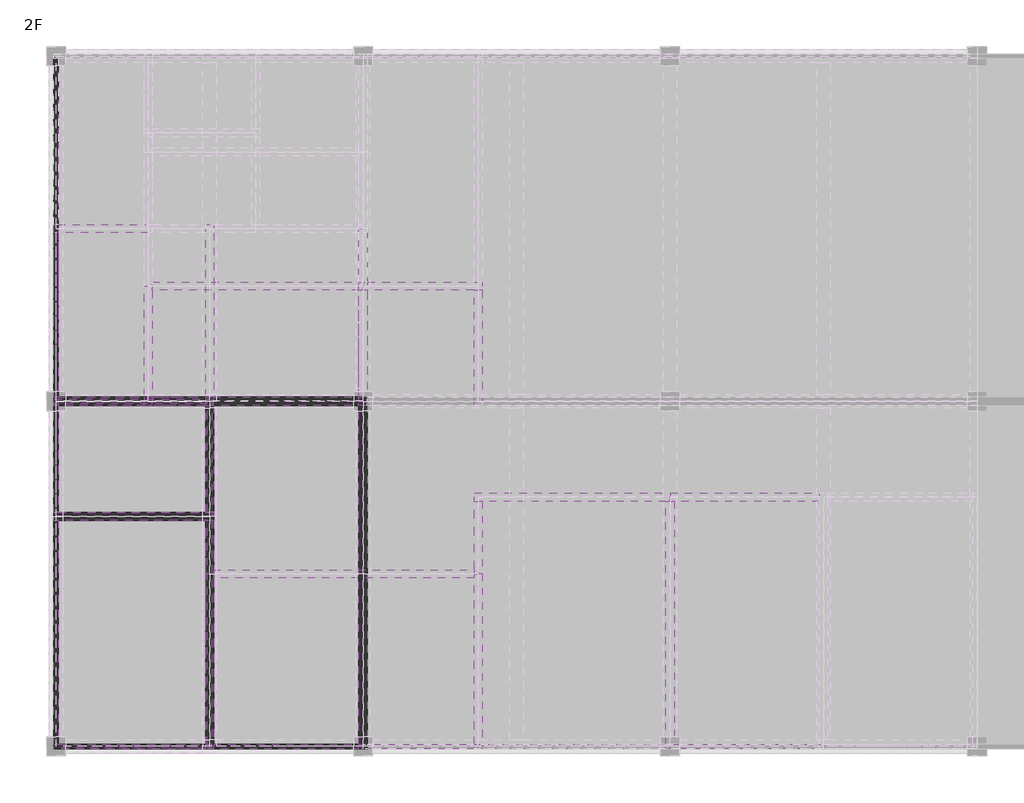
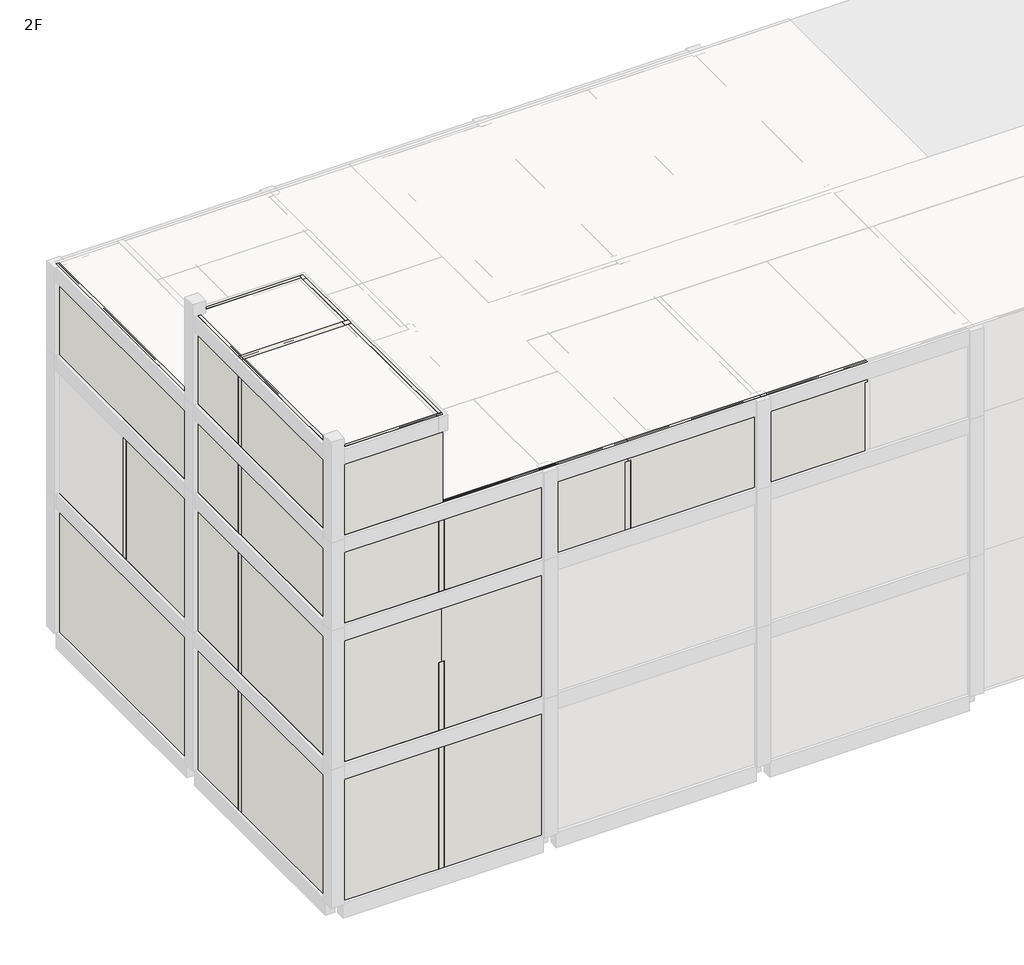
# One storey, part 1 of 7: 56 walls.
"""IFC4 building model written with IfcOpenShell, lengths in millimetres."""

from ifc_helpers import new_model, si_unit, frame, origin, place, context, project, spatial, polyline, outline, extrude, faceted_brep, element, save

model = new_model("IFC4")

# Units and contexts
model_context = context("Model", 3, world=origin())
ifc_project = project(units=[si_unit("LENGTHUNIT", "METRE", prefix="MILLI")], contexts=[model_context])

# Site, building, storey
site = spatial("IfcSite", under=ifc_project)
building = spatial("IfcBuilding", under=site)
storey = spatial("IfcBuildingStorey", under=building, Name="2F", Elevation=3500.0)

# Walls
placement = place(None, origin())
element("IfcWall", 1, ObjectType="WA211_Exterior-Cement Brick-90mm", at=placement, inside=storey, context=model_context, shape_type="SweptSolid", body=[
    extrude(outline(polyline([(45516.6521483, 181866.8614395), (45516.6521483, 173030.8614395), (45402.6521483, 173030.8614395), (45402.6521483, 181866.8614395), (45516.6521483, 181866.8614395)])), frame((0.0, 0.0, 3500.0), z_axis=(0.0, 0.0, 1.0), x_axis=(1.0, 0.0, 0.0)), (0.0, 0.0, 1.0), 5500.0),
])
element("IfcWall", 2, ObjectType="WA211_Exterior-Cement Brick-90mm", at=placement, inside=storey, context=model_context, shape_type="SweptSolid", body=[
    extrude(outline(polyline([(49566.6521483, 163980.8614395), (53352.6521483, 163980.8614395), (53352.6521483, 163866.8614395), (49566.6521483, 163866.8614395), (49566.6521483, 163980.8614395)])), frame((0.0, 0.0, 3500.0), z_axis=(0.0, 0.0, 1.0), x_axis=(1.0, 0.0, 0.0)), (0.0, 0.0, 1.0), 5500.0),
])
element("IfcWall", 3, ObjectType="WA211_Exterior-Cement Brick-90mm", at=placement, inside=storey, context=model_context, shape_type="SweptSolid", body=[
    extrude(outline(polyline([(45516.6521483, 172816.8614395), (45516.6521483, 170030.8614395), (45402.6521483, 170030.8614395), (45402.6521483, 172816.8614395), (45516.6521483, 172816.8614395)])), frame((0.0, 0.0, 3500.0), z_axis=(0.0, 0.0, 1.0), x_axis=(1.0, 0.0, 0.0)), (0.0, 0.0, 1.0), 5500.0),
])
element("IfcWall", 4, ObjectType="WA211_Exterior-Cement Brick-90mm", at=placement, inside=storey, context=model_context, shape_type="SweptSolid", body=[
    extrude(outline(polyline([(45516.6521483, 169816.8614395), (45516.6521483, 163980.8614395), (45402.6521483, 163980.8614395), (45402.6521483, 169816.8614395), (45516.6521483, 169816.8614395)])), frame((0.0, 0.0, 3500.0), z_axis=(0.0, 0.0, 1.0), x_axis=(1.0, 0.0, 0.0)), (0.0, 0.0, 1.0), 5500.0),
])
element("IfcWall", 5, ObjectType="WA211_Exterior-Cement Brick-90mm", at=placement, inside=storey, context=model_context, shape_type="Brep", body=[
    faceted_brep([(49352.6521483, 163980.8614395, 3500.0), (45516.6521483, 163980.8614395, 3500.0), (45402.6521483, 163980.8614395, 3500.0), (45402.6521483, 163980.8614395, 9000.0), (45516.6521483, 163980.8614395, 9000.0), (49352.6521483, 163980.8614395, 9000.0), (49352.6521483, 163866.8614395, 3500.0), (49352.6521483, 163866.8614395, 9000.0), (45402.6521483, 163866.8614395, 9000.0), (45402.6521483, 163866.8614395, 3500.0)], [[[0, 1, 2, 3, 4, 5]], [[6, 7, 8, 9]], [[2, 1, 0, 6, 9]], [[5, 4, 3, 8, 7]], [[0, 5, 7, 6]], [[3, 2, 9, 8]]]),
])
element("IfcWall", 6, ObjectType="WA211_Exterior-Cement Brick-90mm", at=placement, inside=storey, context=model_context, shape_type="SweptSolid", body=[
    extrude(outline(polyline([(45516.6521483, 177316.8614395), (45516.6521483, 173030.8614395), (45402.6521483, 173030.8614395), (45402.6521483, 177316.8614395), (45516.6521483, 177316.8614395)])), frame((0.0, 0.0, 9000.0), z_axis=(0.0, 0.0, 1.0), x_axis=(1.0, 0.0, 0.0)), (0.0, 0.0, 1.0), 5500.0),
])
element("IfcWall", 7, ObjectType="WA211_Exterior-Cement Brick-90mm", at=placement, inside=storey, context=model_context, shape_type="SweptSolid", body=[
    extrude(outline(polyline([(45516.6521483, 172816.8614395), (45516.6521483, 170030.8614395), (45402.6521483, 170030.8614395), (45402.6521483, 172816.8614395), (45516.6521483, 172816.8614395)])), frame((0.0, 0.0, 9000.0), z_axis=(0.0, 0.0, 1.0), x_axis=(1.0, 0.0, 0.0)), (0.0, 0.0, 1.0), 5500.0),
])
element("IfcWall", 8, ObjectType="WA211_Exterior-Cement Brick-90mm", at=placement, inside=storey, context=model_context, shape_type="SweptSolid", body=[
    extrude(outline(polyline([(45516.6521483, 169816.8614395), (45516.6521483, 163980.8614395), (45402.6521483, 163980.8614395), (45402.6521483, 169816.8614395), (45516.6521483, 169816.8614395)])), frame((0.0, 0.0, 9000.0), z_axis=(0.0, 0.0, 1.0), x_axis=(1.0, 0.0, 0.0)), (0.0, 0.0, 1.0), 5500.0),
])
element("IfcWall", 9, ObjectType="WA211_Exterior-Cement Brick-90mm", at=placement, inside=storey, context=model_context, shape_type="Brep", body=[
    faceted_brep([(49352.6521483, 163980.8614395, 9000.0), (45516.6521483, 163980.8614395, 9000.0), (45402.6521483, 163980.8614395, 9000.0), (45402.6521483, 163980.8614395, 14500.0), (45516.6521483, 163980.8614395, 14500.0), (49459.6521483, 163980.8614395, 14500.0), (49459.6521483, 163980.8614395, 11700.0), (49352.6521483, 163980.8614395, 11700.0), (49352.6521483, 163866.8614395, 9000.0), (49352.6521483, 163866.8614395, 11700.0), (49459.6521483, 163866.8614395, 11700.0), (49459.6521483, 163866.8614395, 14500.0), (45402.6521483, 163866.8614395, 14500.0), (45402.6521483, 163866.8614395, 9000.0)], [[[0, 1, 2, 3, 4, 5, 6, 7]], [[8, 9, 10, 11, 12, 13]], [[2, 1, 0, 8, 13]], [[5, 4, 3, 12, 11]], [[3, 2, 13, 12]], [[6, 5, 11, 10]], [[6, 10, 9, 7]], [[0, 7, 9, 8]]]),
])
element("IfcWall", 10, ObjectType="WA211_Exterior-Cement Brick-90mm", at=placement, inside=storey, context=model_context, shape_type="SweptSolid", body=[
    extrude(outline(polyline([(9000.0, 53352.6521483), (12000.0, 53352.6521483), (12000.0, 53459.6521483), (14500.0, 53459.6521483), (14500.0, 49459.6521483), (11700.0, 49459.6521483), (11700.0, 49566.6521483), (9000.0, 49566.6521483), (9000.0, 53352.6521483)])), frame((0.0, 163866.8614395, 0.0), z_axis=(0.0, 1.0, 0.0), x_axis=(0.0, 0.0, 1.0)), (0.0, 0.0, 1.0), 114.0),
])
element("IfcWall", 11, ObjectType="WA211_Exterior-Cement Brick-90mm", at=placement, inside=storey, context=model_context, shape_type="SweptSolid", body=[
    extrude(outline(polyline([(14500.0, 65352.6521483), (17200.0, 65352.6521483), (17200.0, 65459.6521483), (18000.0, 65459.6521483), (18000.0, 61459.6521483), (17200.0, 61459.6521483), (17200.0, 61566.6521483), (14500.0, 61566.6521483), (14500.0, 65352.6521483)])), frame((0.0, 163866.8614395, 0.0), z_axis=(0.0, 1.0, 0.0), x_axis=(0.0, 0.0, 1.0)), (0.0, 0.0, 1.0), 114.0),
])
element("IfcWall", 12, ObjectType="WA211_Exterior-Cement Brick-90mm", at=placement, inside=storey, context=model_context, shape_type="SweptSolid", body=[
    extrude(outline(polyline([(14500.0, 61352.6521483), (17200.0, 61352.6521483), (17200.0, 61459.6521483), (18000.0, 61459.6521483), (18000.0, 56459.6521483), (17200.0, 56459.6521483), (17200.0, 56566.6521483), (14500.0, 56566.6521483), (14500.0, 61352.6521483)])), frame((0.0, 163866.8614395, 0.0), z_axis=(0.0, 1.0, 0.0), x_axis=(0.0, 0.0, 1.0)), (0.0, 0.0, 1.0), 114.0),
])
element("IfcWall", 13, ObjectType="WA211_Exterior-Cement Brick-90mm", at=placement, inside=storey, context=model_context, shape_type="SweptSolid", body=[
    extrude(outline(polyline([(14500.0, 56352.6521483), (17200.0, 56352.6521483), (17200.0, 56459.6521483), (18000.0, 56459.6521483), (18000.0, 49566.6521483), (14500.0, 49566.6521483), (14500.0, 56352.6521483)])), frame((0.0, 163866.8614395, 0.0), z_axis=(0.0, 1.0, 0.0), x_axis=(0.0, 0.0, 1.0)), (0.0, 0.0, 1.0), 114.0),
])
element("IfcWall", 14, ObjectType="WA211_Exterior-Cement Brick-90mm", at=placement, inside=storey, context=model_context, shape_type="SweptSolid", body=[
    extrude(outline(polyline([(45516.6521483, 181866.8614395), (45516.6521483, 173030.8614395), (45402.6521483, 173030.8614395), (45402.6521483, 181866.8614395), (45516.6521483, 181866.8614395)])), frame((0.0, 0.0, 14500.0), z_axis=(0.0, 0.0, 1.0), x_axis=(1.0, 0.0, 0.0)), (0.0, 0.0, 1.0), 3500.0),
])
element("IfcWall", 15, ObjectType="WA211_Exterior-Cement Brick-90mm", at=placement, inside=storey, context=model_context, shape_type="SweptSolid", body=[
    extrude(outline(polyline([(45516.6521483, 172816.8614395), (45516.6521483, 170030.8614395), (45402.6521483, 170030.8614395), (45402.6521483, 172816.8614395), (45516.6521483, 172816.8614395)])), frame((0.0, 0.0, 14500.0), z_axis=(0.0, 0.0, 1.0), x_axis=(1.0, 0.0, 0.0)), (0.0, 0.0, 1.0), 3500.0),
])
element("IfcWall", 16, ObjectType="WA211_Exterior-Cement Brick-90mm", at=placement, inside=storey, context=model_context, shape_type="SweptSolid", body=[
    extrude(outline(polyline([(45516.6521483, 169816.8614395), (45516.6521483, 163980.8614395), (45402.6521483, 163980.8614395), (45402.6521483, 169816.8614395), (45516.6521483, 169816.8614395)])), frame((0.0, 0.0, 14500.0), z_axis=(0.0, 0.0, 1.0), x_axis=(1.0, 0.0, 0.0)), (0.0, 0.0, 1.0), 3500.0),
])
element("IfcWall", 17, ObjectType="WA211_Exterior-Cement Brick-90mm", at=placement, inside=storey, context=model_context, shape_type="Brep", body=[
    faceted_brep([(49352.6521483, 163980.8614395, 14500.0), (45516.6521483, 163980.8614395, 14500.0), (45402.6521483, 163980.8614395, 14500.0), (45402.6521483, 163980.8614395, 18000.0), (45516.6521483, 163980.8614395, 18000.0), (49352.6521483, 163980.8614395, 18000.0), (49352.6521483, 163866.8614395, 14500.0), (49352.6521483, 163866.8614395, 18000.0), (45402.6521483, 163866.8614395, 18000.0), (45402.6521483, 163866.8614395, 14500.0)], [[[0, 1, 2, 3, 4, 5]], [[6, 7, 8, 9]], [[2, 1, 0, 6, 9]], [[5, 4, 3, 8, 7]], [[0, 5, 7, 6]], [[3, 2, 9, 8]]]),
])
element("IfcWall", 18, ObjectType="WA211_Exterior-Cement Brick-90mm", at=placement, inside=storey, context=model_context, shape_type="Brep", body=[
    faceted_brep([(49402.6521483, 172980.8614395, 18000.0), (49402.6521483, 172866.8614395, 18000.0), (49402.6521483, 170030.8614395, 18000.0), (49402.6521483, 170030.8614395, 21500.0), (49402.6521483, 172866.8614395, 21500.0), (49402.6521483, 172980.8614395, 21500.0), (49516.6521483, 172980.8614395, 18000.0), (49516.6521483, 172980.8614395, 21500.0), (49516.6521483, 170030.8614395, 21500.0), (49516.6521483, 170030.8614395, 18000.0)], [[[0, 1, 2, 3, 4, 5]], [[6, 7, 8, 9]], [[2, 1, 0, 6, 9]], [[5, 4, 3, 8, 7]], [[0, 5, 7, 6]], [[3, 2, 9, 8]]]),
])
element("IfcWall", 19, ObjectType="WA211_Exterior-Cement Brick-90mm", at=placement, inside=storey, context=model_context, shape_type="SweptSolid", body=[
    extrude(outline(polyline([(45516.6521483, 172866.8614395), (45516.6521483, 170030.8614395), (45402.6521483, 170030.8614395), (45402.6521483, 172866.8614395), (45516.6521483, 172866.8614395)])), frame((0.0, 0.0, 18000.0), z_axis=(0.0, 0.0, 1.0), x_axis=(1.0, 0.0, 0.0)), (0.0, 0.0, 1.0), 3500.0),
])
element("IfcWall", 20, ObjectType="WA211_Exterior-Cement Brick-90mm", at=placement, inside=storey, context=model_context, shape_type="Brep", body=[
    faceted_brep([(45402.6521483, 172866.8614395, 18000.0), (45516.6521483, 172866.8614395, 18000.0), (49402.6521483, 172866.8614395, 18000.0), (49402.6521483, 172866.8614395, 21500.0), (45516.6521483, 172866.8614395, 21500.0), (45402.6521483, 172866.8614395, 21500.0), (45402.6521483, 172980.8614395, 18000.0), (45402.6521483, 172980.8614395, 21500.0), (49402.6521483, 172980.8614395, 21500.0), (49402.6521483, 172980.8614395, 18000.0)], [[[0, 1, 2, 3, 4, 5]], [[6, 7, 8, 9]], [[2, 1, 0, 6, 9]], [[5, 4, 3, 8, 7]], [[0, 5, 7, 6]], [[3, 2, 9, 8]]]),
])
element("IfcWall", 21, ObjectType="WA211_Exterior-Cement Brick-90mm", at=placement, inside=storey, context=model_context, shape_type="SweptSolid", body=[
    extrude(outline(polyline([(45516.6521483, 169816.8614395), (45516.6521483, 163980.8614395), (45402.6521483, 163980.8614395), (45402.6521483, 169816.8614395), (45516.6521483, 169816.8614395)])), frame((0.0, 0.0, 18000.0), z_axis=(0.0, 0.0, 1.0), x_axis=(1.0, 0.0, 0.0)), (0.0, 0.0, 1.0), 3500.0),
])
element("IfcWall", 22, ObjectType="WA211_Exterior-Cement Brick-90mm", at=placement, inside=storey, context=model_context, shape_type="Brep", body=[
    faceted_brep([(49516.6521483, 163980.8614395, 18000.0), (49402.6521483, 163980.8614395, 18000.0), (45516.6521483, 163980.8614395, 18000.0), (45402.6521483, 163980.8614395, 18000.0), (45402.6521483, 163980.8614395, 21500.0), (45516.6521483, 163980.8614395, 21500.0), (49402.6521483, 163980.8614395, 21500.0), (49516.6521483, 163980.8614395, 21500.0), (49516.6521483, 163866.8614395, 18000.0), (49516.6521483, 163866.8614395, 21500.0), (45402.6521483, 163866.8614395, 21500.0), (45402.6521483, 163866.8614395, 18000.0)], [[[0, 1, 2, 3, 4, 5, 6, 7]], [[8, 9, 10, 11]], [[3, 2, 1, 0, 8, 11]], [[7, 6, 5, 4, 10, 9]], [[4, 3, 11, 10]], [[0, 7, 9, 8]]]),
])
element("IfcWall", 23, ObjectType="WA211_Exterior-Cement Brick-90mm", at=placement, inside=storey, context=model_context, shape_type="SweptSolid", body=[
    extrude(outline(polyline([(49402.6521483, 163980.8614395), (49402.6521483, 169816.8614395), (49516.6521483, 169816.8614395), (49516.6521483, 163980.8614395), (49402.6521483, 163980.8614395)])), frame((0.0, 0.0, 18000.0), z_axis=(0.0, 0.0, 1.0), x_axis=(1.0, 0.0, 0.0)), (0.0, 0.0, 1.0), 3500.0),
])
element("IfcWall", 24, ObjectType="WA221_Interior-Cement Block-190mm", at=placement, inside=storey, context=model_context, shape_type="SweptSolid", body=[
    extrude(outline(polyline([(49566.6521483, 173030.8614395), (53352.6521483, 173030.8614395), (53352.6521483, 172816.8614395), (49566.6521483, 172816.8614395), (49566.6521483, 173030.8614395)])), frame((0.0, 0.0, 3500.0), z_axis=(0.0, 0.0, 1.0), x_axis=(1.0, 0.0, 0.0)), (0.0, 0.0, 1.0), 5500.0),
])
element("IfcWall", 25, ObjectType="WA221_Interior-Cement Block-190mm", at=placement, inside=storey, context=model_context, shape_type="Brep", body=[
    faceted_brep([(45402.6521483, 172816.8614395, 3500.0), (45516.6521483, 172816.8614395, 3500.0), (49352.6521483, 172816.8614395, 3500.0), (49352.6521483, 172816.8614395, 9000.0), (45516.6521483, 172816.8614395, 9000.0), (45402.6521483, 172816.8614395, 9000.0), (45402.6521483, 173030.8614395, 3500.0), (45402.6521483, 173030.8614395, 9000.0), (45516.6521483, 173030.8614395, 9000.0), (49352.6521483, 173030.8614395, 9000.0), (49352.6521483, 173030.8614395, 3500.0), (45516.6521483, 173030.8614395, 3500.0)], [[[0, 1, 2, 3, 4, 5]], [[6, 7, 8, 9, 10, 11]], [[2, 1, 0, 6, 11, 10]], [[5, 4, 3, 9, 8, 7]], [[0, 5, 7, 6]], [[3, 2, 10, 9]]]),
])
element("IfcWall", 26, ObjectType="WA221_Interior-Cement Block-190mm", at=placement, inside=storey, context=model_context, shape_type="Brep", body=[
    faceted_brep([(53566.6521483, 163866.8614395, 3500.0), (53566.6521483, 163980.8614395, 3500.0), (53566.6521483, 172816.8614395, 3500.0), (53566.6521483, 173030.8614395, 3500.0), (53566.6521483, 173030.8614395, 9000.0), (53566.6521483, 172816.8614395, 9000.0), (53566.6521483, 163980.8614395, 9000.0), (53566.6521483, 163866.8614395, 9000.0), (53352.6521483, 163866.8614395, 3500.0), (53352.6521483, 163866.8614395, 9000.0), (53352.6521483, 163980.8614395, 9000.0), (53352.6521483, 172816.8614395, 9000.0), (53352.6521483, 173030.8614395, 9000.0), (53352.6521483, 173030.8614395, 3500.0), (53352.6521483, 172816.8614395, 3500.0), (53352.6521483, 163980.8614395, 3500.0)], [[[0, 1, 2, 3, 4, 5, 6, 7]], [[8, 9, 10, 11, 12, 13, 14, 15]], [[3, 2, 1, 0, 8, 15, 14, 13]], [[7, 6, 5, 4, 12, 11, 10, 9]], [[0, 7, 9, 8]], [[4, 3, 13, 12]]]),
])
element("IfcWall", 27, ObjectType="WA221_Interior-Cement Block-190mm", at=placement, inside=storey, context=model_context, shape_type="Brep", body=[
    faceted_brep([(49352.6521483, 173030.8614395, 3500.0), (49352.6521483, 172816.8614395, 3500.0), (49352.6521483, 170030.8614395, 3500.0), (49352.6521483, 170030.8614395, 9000.0), (49352.6521483, 172816.8614395, 9000.0), (49352.6521483, 173030.8614395, 9000.0), (49566.6521483, 173030.8614395, 3500.0), (49566.6521483, 173030.8614395, 9000.0), (49566.6521483, 172816.8614395, 9000.0), (49566.6521483, 170030.8614395, 9000.0), (49566.6521483, 170030.8614395, 3500.0), (49566.6521483, 172816.8614395, 3500.0)], [[[0, 1, 2, 3, 4, 5]], [[6, 7, 8, 9, 10, 11]], [[2, 1, 0, 6, 11, 10]], [[5, 4, 3, 9, 8, 7]], [[0, 5, 7, 6]], [[3, 2, 10, 9]]]),
])
element("IfcWall", 28, ObjectType="WA221_Interior-Cement Block-190mm", at=placement, inside=storey, context=model_context, shape_type="Brep", body=[
    faceted_brep([(49352.6521483, 169816.8614395, 3500.0), (49352.6521483, 163980.8614395, 3500.0), (49352.6521483, 163866.8614395, 3500.0), (49352.6521483, 163866.8614395, 9000.0), (49352.6521483, 163980.8614395, 9000.0), (49352.6521483, 169816.8614395, 9000.0), (49566.6521483, 169816.8614395, 3500.0), (49566.6521483, 169816.8614395, 9000.0), (49566.6521483, 163980.8614395, 9000.0), (49566.6521483, 163866.8614395, 9000.0), (49566.6521483, 163866.8614395, 3500.0), (49566.6521483, 163980.8614395, 3500.0)], [[[0, 1, 2, 3, 4, 5]], [[6, 7, 8, 9, 10, 11]], [[2, 1, 0, 6, 11, 10]], [[5, 4, 3, 9, 8, 7]], [[3, 2, 10, 9]], [[0, 5, 7, 6]]]),
])
element("IfcWall", 29, ObjectType="WA221_Interior-Cement Block-190mm", at=placement, inside=storey, context=model_context, shape_type="Brep", body=[
    faceted_brep([(45402.6521483, 169816.8614395, 3500.0), (45516.6521483, 169816.8614395, 3500.0), (49352.6521483, 169816.8614395, 3500.0), (49566.6521483, 169816.8614395, 3500.0), (49566.6521483, 169816.8614395, 9000.0), (49352.6521483, 169816.8614395, 9000.0), (45516.6521483, 169816.8614395, 9000.0), (45402.6521483, 169816.8614395, 9000.0), (45402.6521483, 170030.8614395, 3500.0), (45402.6521483, 170030.8614395, 9000.0), (45516.6521483, 170030.8614395, 9000.0), (49352.6521483, 170030.8614395, 9000.0), (49566.6521483, 170030.8614395, 9000.0), (49566.6521483, 170030.8614395, 3500.0), (49352.6521483, 170030.8614395, 3500.0), (45516.6521483, 170030.8614395, 3500.0)], [[[0, 1, 2, 3, 4, 5, 6, 7]], [[8, 9, 10, 11, 12, 13, 14, 15]], [[3, 2, 1, 0, 8, 15, 14, 13]], [[7, 6, 5, 4, 12, 11, 10, 9]], [[0, 7, 9, 8]], [[4, 3, 13, 12]]]),
])
element("IfcWall", 30, ObjectType="WA221_Interior-Cement Block-190mm", at=placement, inside=storey, context=model_context, shape_type="Brep", body=[
    faceted_brep([(53566.6521483, 172923.8614395, 9000.0), (53566.6521483, 173030.8614395, 9000.0), (53566.6521483, 177316.8614395, 9000.0), (53566.6521483, 177316.8614395, 11700.0), (53566.6521483, 177423.8614395, 11700.0), (53566.6521483, 177423.8614395, 12400.0), (53566.6521483, 173030.8614395, 12400.0), (53566.6521483, 172816.8614395, 12400.0), (53566.6521483, 172816.8614395, 12000.0), (53566.6521483, 172923.8614395, 12000.0), (53352.6521483, 172923.8614395, 9000.0), (53352.6521483, 172923.8614395, 12000.0), (53352.6521483, 172816.8614395, 12000.0), (53352.6521483, 172816.8614395, 12400.0), (53352.6521483, 177423.8614395, 12400.0), (53352.6521483, 177423.8614395, 11700.0), (53352.6521483, 177316.8614395, 11700.0), (53352.6521483, 177316.8614395, 9000.0)], [[[0, 1, 2, 3, 4, 5, 6, 7, 8, 9]], [[10, 11, 12, 13, 14, 15, 16, 17]], [[2, 1, 0, 10, 17]], [[7, 6, 5, 14, 13]], [[0, 9, 11, 10]], [[8, 12, 11, 9]], [[8, 7, 13, 12]], [[5, 4, 15, 14]], [[15, 4, 3, 16]], [[3, 2, 17, 16]]]),
])
element("IfcWall", 31, ObjectType="WA221_Interior-Cement Block-190mm", at=placement, inside=storey, context=model_context, shape_type="Brep", body=[
    faceted_brep([(53566.6521483, 163866.8614395, 9000.0), (53566.6521483, 163980.8614395, 9000.0), (53566.6521483, 172816.8614395, 9000.0), (53566.6521483, 172923.8614395, 9000.0), (53566.6521483, 172923.8614395, 12000.0), (53566.6521483, 172816.8614395, 12000.0), (53566.6521483, 163980.8614395, 12000.0), (53566.6521483, 163866.8614395, 12000.0), (53352.6521483, 163866.8614395, 9000.0), (53352.6521483, 163866.8614395, 12000.0), (53352.6521483, 163980.8614395, 12000.0), (53352.6521483, 172816.8614395, 12000.0), (53352.6521483, 172923.8614395, 12000.0), (53352.6521483, 172923.8614395, 9000.0), (53352.6521483, 163980.8614395, 9000.0), (53459.6521483, 163866.8614395, 12000.0)], [[[0, 1, 2, 3, 4, 5, 6, 7]], [[8, 9, 10, 11, 12, 13, 14]], [[3, 2, 1, 0, 8, 14, 13]], [[4, 3, 13, 12]], [[7, 6, 5, 4, 12, 11, 10, 9, 15]], [[0, 7, 15, 9, 8]]]),
])
element("IfcWall", 32, ObjectType="WA221_Interior-Cement Block-190mm", at=placement, inside=storey, context=model_context, shape_type="Brep", body=[
    faceted_brep([(47859.6521483, 177530.8614395, 9000.0), (47752.6521483, 177530.8614395, 9000.0), (45516.6521483, 177530.8614395, 9000.0), (45402.6521483, 177530.8614395, 9000.0), (45402.6521483, 177530.8614395, 14500.0), (45516.6521483, 177530.8614395, 14500.0), (47752.6521483, 177530.8614395, 14500.0), (47966.6521483, 177530.8614395, 14500.0), (47966.6521483, 177530.8614395, 11700.0), (47859.6521483, 177530.8614395, 11700.0), (47859.6521483, 177316.8614395, 9000.0), (47859.6521483, 177316.8614395, 11700.0), (47966.6521483, 177316.8614395, 11700.0), (47966.6521483, 177316.8614395, 14500.0), (45516.6521483, 177316.8614395, 14500.0), (45402.6521483, 177316.8614395, 14500.0), (45402.6521483, 177316.8614395, 9000.0), (45516.6521483, 177316.8614395, 9000.0)], [[[0, 1, 2, 3, 4, 5, 6, 7, 8, 9]], [[10, 11, 12, 13, 14, 15, 16, 17]], [[3, 2, 1, 0, 10, 17, 16]], [[7, 6, 5, 4, 15, 14, 13]], [[0, 9, 11, 10]], [[8, 12, 11, 9]], [[8, 7, 13, 12]], [[4, 3, 16, 15]]]),
])
element("IfcWall", 33, ObjectType="WA221_Interior-Cement Block-190mm", at=placement, inside=storey, context=model_context, shape_type="Brep", body=[
    faceted_brep([(45402.6521483, 172816.8614395, 9000.0), (45516.6521483, 172816.8614395, 9000.0), (49352.6521483, 172816.8614395, 9000.0), (49566.6521483, 172816.8614395, 9000.0), (49566.6521483, 172816.8614395, 14500.0), (49352.6521483, 172816.8614395, 14500.0), (45516.6521483, 172816.8614395, 14500.0), (45402.6521483, 172816.8614395, 14500.0), (45402.6521483, 173030.8614395, 9000.0), (45402.6521483, 173030.8614395, 14500.0), (45516.6521483, 173030.8614395, 14500.0), (49566.6521483, 173030.8614395, 14500.0), (49566.6521483, 173030.8614395, 11700.0), (49566.6521483, 173030.8614395, 9000.0), (49352.6521483, 173030.8614395, 9000.0), (45516.6521483, 173030.8614395, 9000.0)], [[[0, 1, 2, 3, 4, 5, 6, 7]], [[8, 9, 10, 11, 12, 13, 14, 15]], [[3, 2, 1, 0, 8, 15, 14, 13]], [[7, 6, 5, 4, 11, 10, 9]], [[0, 7, 9, 8]], [[3, 13, 12, 11, 4]]]),
])
element("IfcWall", 34, ObjectType="WA221_Interior-Cement Block-190mm", at=placement, inside=storey, context=model_context, shape_type="Brep", body=[
    faceted_brep([(49352.6521483, 177530.8614395, 9000.0), (49352.6521483, 177316.8614395, 9000.0), (49352.6521483, 173030.8614395, 9000.0), (49352.6521483, 173030.8614395, 11700.0), (49352.6521483, 177316.8614395, 11700.0), (49352.6521483, 177530.8614395, 11700.0), (49566.6521483, 177530.8614395, 9000.0), (49566.6521483, 177530.8614395, 11700.0), (49566.6521483, 177316.8614395, 11700.0), (49566.6521483, 173030.8614395, 11700.0), (49566.6521483, 173030.8614395, 9000.0), (49566.6521483, 177316.8614395, 9000.0)], [[[0, 1, 2, 3, 4, 5]], [[6, 7, 8, 9, 10, 11]], [[2, 1, 0, 6, 11, 10]], [[5, 4, 3, 9, 8, 7]], [[0, 5, 7, 6]], [[3, 2, 10, 9]]]),
])
element("IfcWall", 35, ObjectType="WA221_Interior-Cement Block-190mm", at=placement, inside=storey, context=model_context, shape_type="Brep", body=[
    faceted_brep([(49566.6521483, 170030.8614395, 14500.0), (49566.6521483, 170030.8614395, 9000.0), (49352.6521483, 170030.8614395, 9000.0), (45516.6521483, 170030.8614395, 9000.0), (45402.6521483, 170030.8614395, 9000.0), (45402.6521483, 170030.8614395, 14500.0), (45516.6521483, 170030.8614395, 14500.0), (49352.6521483, 170030.8614395, 14500.0), (49566.6521483, 169816.8614395, 9000.0), (49566.6521483, 169816.8614395, 11700.0), (49566.6521483, 169816.8614395, 14500.0), (45516.6521483, 169816.8614395, 14500.0), (45402.6521483, 169816.8614395, 14500.0), (45402.6521483, 169816.8614395, 9000.0), (45516.6521483, 169816.8614395, 9000.0), (49352.6521483, 169816.8614395, 9000.0)], [[[0, 1, 2, 3, 4, 5, 6, 7]], [[8, 9, 10, 11, 12, 13, 14, 15]], [[4, 3, 2, 1, 8, 15, 14, 13]], [[0, 7, 6, 5, 12, 11, 10]], [[5, 4, 13, 12]], [[0, 10, 9, 8, 1]]]),
])
element("IfcWall", 36, ObjectType="WA221_Interior-Cement Block-190mm", at=placement, inside=storey, context=model_context, shape_type="SweptSolid", body=[
    extrude(outline(polyline([(49352.6521483, 170030.8614395), (49352.6521483, 172816.8614395), (49566.6521483, 172816.8614395), (49566.6521483, 170030.8614395), (49352.6521483, 170030.8614395)])), frame((0.0, 0.0, 9000.0), z_axis=(0.0, 0.0, 1.0), x_axis=(1.0, 0.0, 0.0)), (0.0, 0.0, 1.0), 5500.0),
])
element("IfcWall", 37, ObjectType="WA221_Interior-Cement Block-190mm", at=placement, inside=storey, context=model_context, shape_type="Brep", body=[
    faceted_brep([(49352.6521483, 169816.8614395, 9000.0), (49352.6521483, 163980.8614395, 9000.0), (49352.6521483, 163866.8614395, 9000.0), (49352.6521483, 163866.8614395, 11700.0), (49352.6521483, 163980.8614395, 11700.0), (49352.6521483, 169816.8614395, 11700.0), (49566.6521483, 169816.8614395, 9000.0), (49566.6521483, 169816.8614395, 11700.0), (49566.6521483, 163980.8614395, 11700.0), (49566.6521483, 163866.8614395, 11700.0), (49566.6521483, 163866.8614395, 9000.0), (49566.6521483, 163980.8614395, 9000.0), (49459.6521483, 163866.8614395, 11700.0)], [[[0, 1, 2, 3, 4, 5]], [[6, 7, 8, 9, 10, 11]], [[2, 1, 0, 6, 11, 10]], [[5, 4, 3, 12, 9, 8, 7]], [[0, 5, 7, 6]], [[3, 2, 10, 9, 12]]]),
])
element("IfcWall", 38, ObjectType="WA221_Interior-Cement Block-190mm", at=placement, inside=storey, context=model_context, shape_type="Brep", body=[
    faceted_brep([(61352.6521483, 170316.8614395, 14500.0), (61352.6521483, 163980.8614395, 14500.0), (61352.6521483, 163866.8614395, 14500.0), (61352.6521483, 163866.8614395, 17200.0), (61352.6521483, 163980.8614395, 17200.0), (61352.6521483, 170316.8614395, 17200.0), (61566.6521483, 170316.8614395, 14500.0), (61566.6521483, 170316.8614395, 17200.0), (61566.6521483, 163980.8614395, 17200.0), (61566.6521483, 163866.8614395, 17200.0), (61566.6521483, 163866.8614395, 14500.0), (61566.6521483, 163980.8614395, 14500.0), (61459.6521483, 170316.8614395, 14500.0), (61459.6521483, 163866.8614395, 17200.0), (61459.6521483, 170316.8614395, 17200.0)], [[[0, 1, 2, 3, 4, 5]], [[6, 7, 8, 9, 10, 11]], [[2, 1, 0, 12, 6, 11, 10]], [[5, 4, 3, 13, 9, 8, 7, 14]], [[3, 2, 10, 9, 13]], [[0, 5, 14, 7, 6, 12]]]),
])
element("IfcWall", 39, ObjectType="WA221_Interior-Cement Block-190mm", at=placement, inside=storey, context=model_context, shape_type="Brep", body=[
    faceted_brep([(61459.6521483, 170316.8614395, 14500.0), (61566.6521483, 170316.8614395, 14500.0), (65352.6521483, 170316.8614395, 14500.0), (65352.6521483, 170316.8614395, 17200.0), (61566.6521483, 170316.8614395, 17200.0), (61459.6521483, 170316.8614395, 17200.0), (61459.6521483, 170530.8614395, 14500.0), (61459.6521483, 170530.8614395, 17200.0), (65352.6521483, 170530.8614395, 17200.0), (65352.6521483, 170530.8614395, 14500.0)], [[[0, 1, 2, 3, 4, 5]], [[6, 7, 8, 9]], [[2, 1, 0, 6, 9]], [[5, 4, 3, 8, 7]], [[0, 5, 7, 6]], [[3, 2, 9, 8]]]),
])
element("IfcWall", 40, ObjectType="WA221_Interior-Cement Block-190mm", at=placement, inside=storey, context=model_context, shape_type="Brep", body=[
    faceted_brep([(56566.6521483, 172816.8614395, 14500.0), (56566.6521483, 173030.8614395, 14500.0), (56566.6521483, 175816.8614395, 14500.0), (56566.6521483, 175816.8614395, 17200.0), (56566.6521483, 173030.8614395, 17200.0), (56566.6521483, 172816.8614395, 17200.0), (56352.6521483, 172816.8614395, 14500.0), (56352.6521483, 172816.8614395, 17200.0), (56352.6521483, 175816.8614395, 17200.0), (56352.6521483, 175816.8614395, 14500.0)], [[[0, 1, 2, 3, 4, 5]], [[6, 7, 8, 9]], [[2, 1, 0, 6, 9]], [[5, 4, 3, 8, 7]], [[0, 5, 7, 6]], [[3, 2, 9, 8]]]),
])
element("IfcWall", 41, ObjectType="WA221_Interior-Cement Block-190mm", at=placement, inside=storey, context=model_context, shape_type="Brep", body=[
    faceted_brep([(56566.6521483, 163866.8614395, 14500.0), (56566.6521483, 163980.8614395, 14500.0), (56566.6521483, 168423.8614395, 14500.0), (56566.6521483, 168423.8614395, 17200.0), (56566.6521483, 163980.8614395, 17200.0), (56566.6521483, 163866.8614395, 17200.0), (56352.6521483, 163866.8614395, 14500.0), (56352.6521483, 163866.8614395, 17200.0), (56352.6521483, 163980.8614395, 17200.0), (56352.6521483, 168316.8614395, 17200.0), (56352.6521483, 168423.8614395, 17200.0), (56352.6521483, 168423.8614395, 14500.0), (56352.6521483, 168316.8614395, 14500.0), (56352.6521483, 163980.8614395, 14500.0), (56459.6521483, 163866.8614395, 17200.0)], [[[0, 1, 2, 3, 4, 5]], [[6, 7, 8, 9, 10, 11, 12, 13]], [[2, 1, 0, 6, 13, 12, 11]], [[3, 2, 11, 10]], [[5, 4, 3, 10, 9, 8, 7, 14]], [[0, 5, 14, 7, 6]]]),
])
element("IfcWall", 42, ObjectType="WA221_Interior-Cement Block-190mm", at=placement, inside=storey, context=model_context, shape_type="Brep", body=[
    faceted_brep([(56352.6521483, 170316.8614395, 14500.0), (56566.6521483, 170316.8614395, 14500.0), (61352.6521483, 170316.8614395, 14500.0), (61459.6521483, 170316.8614395, 14500.0), (61459.6521483, 170316.8614395, 17200.0), (61352.6521483, 170316.8614395, 17200.0), (56566.6521483, 170316.8614395, 17200.0), (56352.6521483, 170316.8614395, 17200.0), (56352.6521483, 170530.8614395, 14500.0), (56352.6521483, 170530.8614395, 17200.0), (61459.6521483, 170530.8614395, 17200.0), (61459.6521483, 170530.8614395, 14500.0)], [[[0, 1, 2, 3, 4, 5, 6, 7]], [[8, 9, 10, 11]], [[3, 2, 1, 0, 8, 11]], [[4, 3, 11, 10]], [[7, 6, 5, 4, 10, 9]], [[0, 7, 9, 8]]]),
])
element("IfcWall", 43, ObjectType="WA221_Interior-Cement Block-190mm", at=placement, inside=storey, context=model_context, shape_type="Brep", body=[
    faceted_brep([(56566.6521483, 168423.8614395, 14500.0), (56566.6521483, 170316.8614395, 14500.0), (56566.6521483, 170316.8614395, 17200.0), (56566.6521483, 168423.8614395, 17200.0), (56352.6521483, 168423.8614395, 14500.0), (56352.6521483, 168423.8614395, 17200.0), (56352.6521483, 168530.8614395, 17200.0), (56352.6521483, 170316.8614395, 17200.0), (56352.6521483, 170316.8614395, 14500.0), (56352.6521483, 168530.8614395, 14500.0)], [[[0, 1, 2, 3]], [[4, 5, 6, 7, 8, 9]], [[1, 0, 4, 9, 8]], [[3, 2, 7, 6, 5]], [[0, 3, 5, 4]], [[2, 1, 8, 7]]]),
])
element("IfcWall", 44, ObjectType="WA221_Interior-Cement Block-190mm", at=placement, inside=storey, context=model_context, shape_type="Brep", body=[
    faceted_brep([(49352.6521483, 168423.8614395, 18000.0), (49352.6521483, 168423.8614395, 14500.0), (49352.6521483, 163980.8614395, 14500.0), (49352.6521483, 163866.8614395, 14500.0), (49352.6521483, 163866.8614395, 18000.0), (49352.6521483, 163980.8614395, 18000.0), (49566.6521483, 168423.8614395, 14500.0), (49566.6521483, 168423.8614395, 18000.0), (49566.6521483, 163980.8614395, 18000.0), (49566.6521483, 163866.8614395, 18000.0), (49566.6521483, 163866.8614395, 14500.0), (49566.6521483, 163980.8614395, 14500.0), (49566.6521483, 168316.8614395, 14500.0)], [[[0, 1, 2, 3, 4, 5]], [[6, 7, 8, 9, 10, 11, 12]], [[3, 2, 1, 6, 12, 11, 10]], [[0, 5, 4, 9, 8, 7]], [[0, 7, 6, 1]], [[4, 3, 10, 9]]]),
])
element("IfcWall", 45, ObjectType="WA221_Interior-Cement Block-190mm", at=placement, inside=storey, context=model_context, shape_type="Brep", body=[
    faceted_brep([(56352.6521483, 168530.8614395, 14500.0), (49566.6521483, 168530.8614395, 14500.0), (49566.6521483, 168530.8614395, 17200.0), (56352.6521483, 168530.8614395, 17200.0), (56352.6521483, 168316.8614395, 14500.0), (56352.6521483, 168316.8614395, 17200.0), (49566.6521483, 168316.8614395, 17200.0), (49566.6521483, 168316.8614395, 14500.0), (56352.6521483, 168423.8614395, 14500.0), (49566.6521483, 168423.8614395, 14500.0), (56352.6521483, 168423.8614395, 17200.0)], [[[0, 1, 2, 3]], [[4, 5, 6, 7]], [[1, 0, 8, 4, 7, 9]], [[3, 2, 6, 5, 10]], [[0, 3, 10, 5, 4, 8]], [[2, 1, 9, 7, 6]]]),
])
element("IfcWall", 46, ObjectType="WA221_Interior-Cement Block-190mm", at=placement, inside=storey, context=model_context, shape_type="Brep", body=[
    faceted_brep([(47966.6521483, 175816.8614395, 14500.0), (53352.6521483, 175816.8614395, 14500.0), (53459.6521483, 175816.8614395, 14500.0), (53459.6521483, 175816.8614395, 17200.0), (53352.6521483, 175816.8614395, 17200.0), (47966.6521483, 175816.8614395, 17200.0), (47966.6521483, 176030.8614395, 14500.0), (47966.6521483, 176030.8614395, 17200.0), (53352.6521483, 176030.8614395, 17200.0), (53459.6521483, 176030.8614395, 17200.0), (53459.6521483, 176030.8614395, 14500.0), (53352.6521483, 176030.8614395, 14500.0), (47966.6521483, 175923.8614395, 14500.0)], [[[0, 1, 2, 3, 4, 5]], [[6, 7, 8, 9, 10, 11]], [[2, 1, 0, 12, 6, 11, 10]], [[3, 2, 10, 9]], [[5, 4, 3, 9, 8, 7]], [[0, 5, 7, 6, 12]]]),
])
element("IfcWall", 47, ObjectType="WA221_Interior-Cement Block-190mm", at=placement, inside=storey, context=model_context, shape_type="Brep", body=[
    faceted_brep([(53459.6521483, 175816.8614395, 14500.0), (53566.6521483, 175816.8614395, 14500.0), (56352.6521483, 175816.8614395, 14500.0), (56566.6521483, 175816.8614395, 14500.0), (56566.6521483, 175816.8614395, 17200.0), (56352.6521483, 175816.8614395, 17200.0), (53566.6521483, 175816.8614395, 17200.0), (53459.6521483, 175816.8614395, 17200.0), (53459.6521483, 176030.8614395, 14500.0), (53459.6521483, 176030.8614395, 17200.0), (53566.6521483, 176030.8614395, 17200.0), (56352.6521483, 176030.8614395, 17200.0), (56566.6521483, 176030.8614395, 17200.0), (56566.6521483, 176030.8614395, 14500.0), (56352.6521483, 176030.8614395, 14500.0), (53566.6521483, 176030.8614395, 14500.0)], [[[0, 1, 2, 3, 4, 5, 6, 7]], [[8, 9, 10, 11, 12, 13, 14, 15]], [[3, 2, 1, 0, 8, 15, 14, 13]], [[7, 6, 5, 4, 12, 11, 10, 9]], [[0, 7, 9, 8]], [[4, 3, 13, 12]]]),
])
element("IfcWall", 48, ObjectType="WA221_Interior-Cement Block-190mm", at=placement, inside=storey, context=model_context, shape_type="Brep", body=[
    faceted_brep([(47752.6521483, 175923.8614395, 18000.0), (47752.6521483, 175923.8614395, 14500.0), (47752.6521483, 173030.8614395, 14500.0), (47752.6521483, 172816.8614395, 14500.0), (47752.6521483, 172816.8614395, 18000.0), (47752.6521483, 173030.8614395, 18000.0), (47966.6521483, 175923.8614395, 14500.0), (47966.6521483, 175923.8614395, 18000.0), (47966.6521483, 173030.8614395, 18000.0), (47966.6521483, 172816.8614395, 18000.0), (47966.6521483, 172816.8614395, 14500.0), (47966.6521483, 173030.8614395, 14500.0), (47966.6521483, 175816.8614395, 14500.0)], [[[0, 1, 2, 3, 4, 5]], [[6, 7, 8, 9, 10, 11, 12]], [[3, 2, 1, 6, 12, 11, 10]], [[0, 5, 4, 9, 8, 7]], [[0, 7, 6, 1]], [[4, 3, 10, 9]]]),
])
element("IfcWall", 49, ObjectType="WA221_Interior-Cement Block-190mm", at=placement, inside=storey, context=model_context, shape_type="SweptSolid", body=[
    extrude(outline(polyline([(49352.6521483, 172816.8614395), (47966.6521483, 172816.8614395), (47966.6521483, 173030.8614395), (49352.6521483, 173030.8614395), (49352.6521483, 172816.8614395)])), frame((0.0, 0.0, 14500.0), z_axis=(0.0, 0.0, 1.0), x_axis=(1.0, 0.0, 0.0)), (0.0, 0.0, 1.0), 3500.0),
])
element("IfcWall", 50, ObjectType="WA221_Interior-Cement Block-190mm", at=placement, inside=storey, context=model_context, shape_type="Brep", body=[
    faceted_brep([(53566.6521483, 173030.8614395, 14500.0), (53352.6521483, 173030.8614395, 14500.0), (49566.6521483, 173030.8614395, 14500.0), (49566.6521483, 173030.8614395, 17200.0), (53352.6521483, 173030.8614395, 17200.0), (53566.6521483, 173030.8614395, 17200.0), (53566.6521483, 172816.8614395, 14500.0), (53566.6521483, 172816.8614395, 17200.0), (49566.6521483, 172816.8614395, 17200.0), (49566.6521483, 172816.8614395, 14500.0)], [[[0, 1, 2, 3, 4, 5]], [[6, 7, 8, 9]], [[2, 1, 0, 6, 9]], [[5, 4, 3, 8, 7]], [[0, 5, 7, 6]], [[3, 2, 9, 8]]]),
])
element("IfcWall", 51, ObjectType="WA221_Interior-Cement Block-190mm", at=placement, inside=storey, context=model_context, shape_type="Brep", body=[
    faceted_brep([(53352.6521483, 175816.8614395, 14500.0), (53352.6521483, 173030.8614395, 14500.0), (53352.6521483, 173030.8614395, 17200.0), (53352.6521483, 175816.8614395, 17200.0), (53566.6521483, 175816.8614395, 14500.0), (53566.6521483, 175816.8614395, 17200.0), (53566.6521483, 173030.8614395, 17200.0), (53566.6521483, 173030.8614395, 14500.0), (53459.6521483, 175816.8614395, 14500.0), (53459.6521483, 175816.8614395, 17200.0)], [[[0, 1, 2, 3]], [[4, 5, 6, 7]], [[1, 0, 8, 4, 7]], [[3, 2, 6, 5, 9]], [[0, 3, 9, 5, 4, 8]], [[2, 1, 7, 6]]]),
])
element("IfcWall", 52, ObjectType="WA221_Interior-Cement Block-190mm", at=placement, inside=storey, context=model_context, shape_type="Brep", body=[
    faceted_brep([(47752.6521483, 173030.8614395, 14500.0), (45516.6521483, 173030.8614395, 14500.0), (45402.6521483, 173030.8614395, 14500.0), (45402.6521483, 173030.8614395, 18000.0), (45516.6521483, 173030.8614395, 18000.0), (47752.6521483, 173030.8614395, 18000.0), (47752.6521483, 172816.8614395, 14500.0), (47752.6521483, 172816.8614395, 18000.0), (45516.6521483, 172816.8614395, 18000.0), (45402.6521483, 172816.8614395, 18000.0), (45402.6521483, 172816.8614395, 14500.0), (45516.6521483, 172816.8614395, 14500.0)], [[[0, 1, 2, 3, 4, 5]], [[6, 7, 8, 9, 10, 11]], [[2, 1, 0, 6, 11, 10]], [[5, 4, 3, 9, 8, 7]], [[0, 5, 7, 6]], [[3, 2, 10, 9]]]),
])
element("IfcWall", 53, ObjectType="WA221_Interior-Cement Block-190mm", at=placement, inside=storey, context=model_context, shape_type="Brep", body=[
    faceted_brep([(45402.6521483, 169816.8614395, 14500.0), (45516.6521483, 169816.8614395, 14500.0), (49352.6521483, 169816.8614395, 14500.0), (49566.6521483, 169816.8614395, 14500.0), (49566.6521483, 169816.8614395, 18000.0), (49352.6521483, 169816.8614395, 18000.0), (45516.6521483, 169816.8614395, 18000.0), (45402.6521483, 169816.8614395, 18000.0), (45402.6521483, 170030.8614395, 14500.0), (45402.6521483, 170030.8614395, 18000.0), (45516.6521483, 170030.8614395, 18000.0), (49352.6521483, 170030.8614395, 18000.0), (49566.6521483, 170030.8614395, 18000.0), (49566.6521483, 170030.8614395, 14500.0), (49352.6521483, 170030.8614395, 14500.0), (45516.6521483, 170030.8614395, 14500.0)], [[[0, 1, 2, 3, 4, 5, 6, 7]], [[8, 9, 10, 11, 12, 13, 14, 15]], [[3, 2, 1, 0, 8, 15, 14, 13]], [[7, 6, 5, 4, 12, 11, 10, 9]], [[0, 7, 9, 8]], [[4, 3, 13, 12]]]),
])
element("IfcWall", 54, ObjectType="WA221_Interior-Cement Block-190mm", at=placement, inside=storey, context=model_context, shape_type="Brep", body=[
    faceted_brep([(49352.6521483, 173030.8614395, 18000.0), (49352.6521483, 173030.8614395, 14500.0), (49352.6521483, 172816.8614395, 14500.0), (49352.6521483, 170030.8614395, 14500.0), (49352.6521483, 170030.8614395, 18000.0), (49352.6521483, 172816.8614395, 18000.0), (49566.6521483, 173030.8614395, 14500.0), (49566.6521483, 173030.8614395, 17200.0), (49566.6521483, 173030.8614395, 18000.0), (49566.6521483, 170030.8614395, 18000.0), (49566.6521483, 170030.8614395, 14500.0), (49566.6521483, 172816.8614395, 14500.0)], [[[0, 1, 2, 3, 4, 5]], [[6, 7, 8, 9, 10, 11]], [[3, 2, 1, 6, 11, 10]], [[0, 5, 4, 9, 8]], [[4, 3, 10, 9]], [[0, 8, 7, 6, 1]]]),
])
element("IfcWall", 55, ObjectType="WA221_Interior-Cement Block-190mm", at=placement, inside=storey, context=model_context, shape_type="Brep", body=[
    faceted_brep([(49352.6521483, 169816.8614395, 14500.0), (49352.6521483, 168423.8614395, 14500.0), (49352.6521483, 168423.8614395, 18000.0), (49352.6521483, 169816.8614395, 18000.0), (49566.6521483, 169816.8614395, 14500.0), (49566.6521483, 169816.8614395, 18000.0), (49566.6521483, 168423.8614395, 18000.0), (49566.6521483, 168423.8614395, 14500.0), (49566.6521483, 168530.8614395, 14500.0)], [[[0, 1, 2, 3]], [[4, 5, 6, 7, 8]], [[1, 0, 4, 8, 7]], [[3, 2, 6, 5]], [[1, 7, 6, 2]], [[0, 3, 5, 4]]]),
])
element("IfcWall", 56, ObjectType="WA221_Interior-Cement Block-190mm", at=placement, inside=storey, context=model_context, shape_type="Brep", body=[
    faceted_brep([(49516.6521483, 170030.8614395, 18000.0), (49402.6521483, 170030.8614395, 18000.0), (45516.6521483, 170030.8614395, 18000.0), (45402.6521483, 170030.8614395, 18000.0), (45402.6521483, 170030.8614395, 21500.0), (45516.6521483, 170030.8614395, 21500.0), (49402.6521483, 170030.8614395, 21500.0), (49516.6521483, 170030.8614395, 21500.0), (49516.6521483, 169816.8614395, 18000.0), (49516.6521483, 169816.8614395, 21500.0), (49402.6521483, 169816.8614395, 21500.0), (45516.6521483, 169816.8614395, 21500.0), (45402.6521483, 169816.8614395, 21500.0), (45402.6521483, 169816.8614395, 18000.0), (45516.6521483, 169816.8614395, 18000.0), (49402.6521483, 169816.8614395, 18000.0)], [[[0, 1, 2, 3, 4, 5, 6, 7]], [[8, 9, 10, 11, 12, 13, 14, 15]], [[3, 2, 1, 0, 8, 15, 14, 13]], [[7, 6, 5, 4, 12, 11, 10, 9]], [[0, 7, 9, 8]], [[4, 3, 13, 12]]]),
])

save(model, "model.ifc")

# Revit data of these elements
# Type "WA211_Exterior-Cement Brick-90mm"
#   Type Comments = ""
#   Layers, outside or top first: 0 mm "A04AL081-00001_Skirt_Acrylic Emulsion Paint" (function 100); 0 mm "A04AL077-00001_Ext Wall Painting_Acrylic Emulsion Paint" (function 100); 12 mm "A04AS164-00001_Plastering_Ext" (function 4); 90 mm "A04AK073-00001_Concrete Brick_0.5B" (function 1); 12 mm "A04AS164-00002_Plastering_Int" (function 5); 0 mm "A04AL078-00002_Int Wall Painting_Water Emulsion Paint" (function 100); 0 mm "A04AL081-00001_Skirt_Acrylic Emulsion Paint" (function 100)
# Type "WA221_Interior-Cement Block-190mm"
#   Type Comments = ""
#   Layers, outside or top first: 0 mm "A04AL081-00001_Skirt_Acrylic Emulsion Paint" (function 100); 0 mm "A04AL078-00002_Int Wall Painting_Water Emulsion Paint" (function 100); 12 mm "A04AS164-00002_Plastering_Int" (function 2); 190 mm "A04AK069-00002_Reinforced Concrete Block_THK 100-200mm" (function 1); 12 mm "A04AS164-00002_Plastering_Int" (function 2); 0 mm "A04AL078-00002_Int Wall Painting_Water Emulsion Paint" (function 100); 0 mm "A04AL081-00001_Skirt_Acrylic Emulsion Paint" (function 100)
# Elements 1, 2, 3, 4 (IfcWall, "WA211_Exterior-Cement Brick-90mm")
#   Top Offset = 0 mm
#   Base Offset = 0 mm
#   Unconnected Height = 5500 mm
#   wall height = 5500 mm
#   Phase Created = New Construction
#   Base Constraint = 2F
#   Materials on its faces: "Default Wall", "A04AS164-00002_Plastering_Int", "A04AS164-00001_Plastering_Ext"
# Element 5 (IfcWall, "WA211_Exterior-Cement Brick-90mm")
#   Top Offset = 0 mm
#   Base Offset = 0 mm
#   Unconnected Height = 5500 mm
#   wall height = 5500 mm
#   Phase Created = New Construction
#   Base Constraint = 2F
#   Materials on its faces: "Default Wall", "A04AS164-00001_Plastering_Ext", "A04AS164-00002_Plastering_Int"
# Elements 6, 7, 8, 10 (IfcWall, "WA211_Exterior-Cement Brick-90mm")
#   Top Offset = 0 mm
#   Base Offset = 0 mm
#   Unconnected Height = 5500 mm
#   wall height = 5500 mm
#   Phase Created = New Construction
#   Base Constraint = 3F
#   Materials on its faces: "Default Wall", "A04AS164-00002_Plastering_Int", "A04AS164-00001_Plastering_Ext"
# Element 9 (IfcWall, "WA211_Exterior-Cement Brick-90mm")
#   Top Offset = 0 mm
#   Base Offset = 0 mm
#   Unconnected Height = 5500 mm
#   wall height = 5500 mm
#   Phase Created = New Construction
#   Base Constraint = 3F
#   Materials on its faces: "Default Wall", "A04AS164-00001_Plastering_Ext", "A04AS164-00002_Plastering_Int"
# Elements 11, 12, 13, 14, 15, 16 (IfcWall, "WA211_Exterior-Cement Brick-90mm")
#   Top Offset = 0 mm
#   Base Offset = 0 mm
#   Unconnected Height = 3500 mm
#   wall height = 3500 mm
#   Phase Created = New Construction
#   Base Constraint = 4F
#   Materials on its faces: "Default Wall", "A04AS164-00002_Plastering_Int", "A04AS164-00001_Plastering_Ext"
# Element 17 (IfcWall, "WA211_Exterior-Cement Brick-90mm")
#   Top Offset = 0 mm
#   Base Offset = 0 mm
#   Unconnected Height = 3500 mm
#   wall height = 3500 mm
#   Phase Created = New Construction
#   Base Constraint = 4F
#   Materials on its faces: "Default Wall", "A04AS164-00001_Plastering_Ext", "A04AS164-00002_Plastering_Int"
# Elements 18, 20 (IfcWall, "WA211_Exterior-Cement Brick-90mm")
#   Top Offset = 0 mm
#   Base Offset = 0 mm
#   Unconnected Height = 3500 mm
#   wall height = 3500 mm
#   Phase Created = New Construction
#   Base Constraint = PF
#   Materials on its faces: "Default Wall", "A04AS164-00001_Plastering_Ext", "A04AS164-00002_Plastering_Int"
# Elements 19, 21, 23 (IfcWall, "WA211_Exterior-Cement Brick-90mm")
#   Top Offset = 0 mm
#   Base Offset = 0 mm
#   Unconnected Height = 3500 mm
#   wall height = 3500 mm
#   Phase Created = New Construction
#   Base Constraint = PF
#   Materials on its faces: "Default Wall", "A04AS164-00002_Plastering_Int", "A04AS164-00001_Plastering_Ext"
# Element 22 (IfcWall, "WA211_Exterior-Cement Brick-90mm")
#   Top Offset = 0 mm
#   Base Offset = 0 mm
#   Unconnected Height = 3500 mm
#   wall height = 3500 mm
#   Phase Created = New Construction
#   Base Constraint = PF
#   Materials on its faces: "A04AS164-00001_Plastering_Ext", "Default Wall", "A04AS164-00002_Plastering_Int"
# Element 24 (IfcWall, "WA221_Interior-Cement Block-190mm")
#   Top Offset = 0 mm
#   Base Offset = 0 mm
#   Unconnected Height = 5500 mm
#   wall height = 5500 mm
#   Phase Created = New Construction
#   Base Constraint = 2F
#   Materials on its faces: "Default Wall", "A04AS164-00002_Plastering_Int"
# Elements 25, 28 (IfcWall, "WA221_Interior-Cement Block-190mm")
#   Top Offset = 0 mm
#   Base Offset = 0 mm
#   Unconnected Height = 5500 mm
#   wall height = 5500 mm
#   Phase Created = New Construction
#   Base Constraint = 2F
#   Materials on its faces: "Default Wall", "A04AS164-00002_Plastering_Int", "A04AS164-00001_Plastering_Ext"
# Elements 26, 29 (IfcWall, "WA221_Interior-Cement Block-190mm")
#   Top Offset = 0 mm
#   Base Offset = 0 mm
#   Unconnected Height = 5500 mm
#   wall height = 5500 mm
#   Phase Created = New Construction
#   Base Constraint = 2F
#   Materials on its faces: "A04AS164-00002_Plastering_Int", "Default Wall", "A04AS164-00001_Plastering_Ext"
# Element 27 (IfcWall, "WA221_Interior-Cement Block-190mm")
#   Top Offset = 0 mm
#   Base Offset = 0 mm
#   Unconnected Height = 5500 mm
#   wall height = 5500 mm
#   Phase Created = New Construction
#   Base Constraint = 2F
#   Materials on its faces: "A04AS164-00002_Plastering_Int", "Default Wall"
# Element 30 (IfcWall, "WA221_Interior-Cement Block-190mm")
#   Top Offset = 0 mm
#   Base Offset = 0 mm
#   Unconnected Height = 3400 mm
#   wall height = 3400 mm
#   Phase Created = New Construction
#   Base Constraint = 3F
#   Materials on its faces: "Default Wall", "A04AS164-00002_Plastering_Int"
# Element 31 (IfcWall, "WA221_Interior-Cement Block-190mm")
#   Top Offset = 0 mm
#   Base Offset = 0 mm
#   Unconnected Height = 3000 mm
#   wall height = 3000 mm
#   Phase Created = New Construction
#   Base Constraint = 3F
#   Materials on its faces: "Default Wall", "A04AS164-00002_Plastering_Int", "A04AS164-00001_Plastering_Ext"
# Element 32 (IfcWall, "WA221_Interior-Cement Block-190mm")
#   Top Offset = 0 mm
#   Base Offset = 0 mm
#   Unconnected Height = 5500 mm
#   wall height = 5500 mm
#   Phase Created = New Construction
#   Base Constraint = 3F
#   Materials on its faces: "Default Wall", "A04AS164-00002_Plastering_Int", "A04AS164-00001_Plastering_Ext"
# Elements 33, 35 (IfcWall, "WA221_Interior-Cement Block-190mm")
#   Top Offset = 0 mm
#   Base Offset = 0 mm
#   Unconnected Height = 5500 mm
#   wall height = 5500 mm
#   Phase Created = New Construction
#   Base Constraint = 3F
#   Materials on its faces: "A04AS164-00002_Plastering_Int", "Default Wall", "A04AS164-00001_Plastering_Ext"
# Element 34 (IfcWall, "WA221_Interior-Cement Block-190mm")
#   Top Offset = 0 mm
#   Base Offset = 0 mm
#   Unconnected Height = 2700 mm
#   wall height = 2700 mm
#   Phase Created = New Construction
#   Base Constraint = 3F
#   Materials on its faces: "A04AS164-00002_Plastering_Int", "Default Wall"
# Element 36 (IfcWall, "WA221_Interior-Cement Block-190mm")
#   Top Offset = 0 mm
#   Base Offset = 0 mm
#   Unconnected Height = 5500 mm
#   wall height = 5500 mm
#   Phase Created = New Construction
#   Base Constraint = 3F
#   Materials on its faces: "Default Wall", "A04AS164-00002_Plastering_Int"
# Element 37 (IfcWall, "WA221_Interior-Cement Block-190mm")
#   Top Offset = 0 mm
#   Base Offset = 0 mm
#   Unconnected Height = 2700 mm
#   wall height = 2700 mm
#   Phase Created = New Construction
#   Base Constraint = 3F
#   Materials on its faces: "Default Wall", "A04AS164-00002_Plastering_Int", "A04AS164-00001_Plastering_Ext"
# Elements 38, 41 (IfcWall, "WA221_Interior-Cement Block-190mm")
#   Top Offset = 0 mm
#   Base Offset = 0 mm
#   Unconnected Height = 2700 mm
#   wall height = 2700 mm
#   Phase Created = New Construction
#   Base Constraint = 4F
#   Materials on its faces: "Default Wall", "A04AS164-00002_Plastering_Int", "A04AS164-00001_Plastering_Ext"
# Elements 39, 43, 45, 46, 51 (IfcWall, "WA221_Interior-Cement Block-190mm")
#   Top Offset = 0 mm
#   Base Offset = 0 mm
#   Unconnected Height = 2700 mm
#   wall height = 2700 mm
#   Phase Created = New Construction
#   Base Constraint = 4F
#   Materials on its faces: "Default Wall", "A04AS164-00002_Plastering_Int"
# Elements 40, 42, 47, 50 (IfcWall, "WA221_Interior-Cement Block-190mm")
#   Top Offset = 0 mm
#   Base Offset = 0 mm
#   Unconnected Height = 2700 mm
#   wall height = 2700 mm
#   Phase Created = New Construction
#   Base Constraint = 4F
#   Materials on its faces: "A04AS164-00002_Plastering_Int", "Default Wall"
# Elements 44, 52 (IfcWall, "WA221_Interior-Cement Block-190mm")
#   Top Offset = 0 mm
#   Base Offset = 0 mm
#   Unconnected Height = 3500 mm
#   wall height = 3500 mm
#   Phase Created = New Construction
#   Base Constraint = 4F
#   Materials on its faces: "Default Wall", "A04AS164-00002_Plastering_Int", "A04AS164-00001_Plastering_Ext"
# Elements 48, 54 (IfcWall, "WA221_Interior-Cement Block-190mm")
#   Top Offset = 0 mm
#   Base Offset = 0 mm
#   Unconnected Height = 3500 mm
#   wall height = 3500 mm
#   Phase Created = New Construction
#   Base Constraint = 4F
#   Materials on its faces: "A04AS164-00002_Plastering_Int", "Default Wall"
# Elements 49, 55 (IfcWall, "WA221_Interior-Cement Block-190mm")
#   Top Offset = 0 mm
#   Base Offset = 0 mm
#   Unconnected Height = 3500 mm
#   wall height = 3500 mm
#   Phase Created = New Construction
#   Base Constraint = 4F
#   Materials on its faces: "Default Wall", "A04AS164-00002_Plastering_Int"
# Element 53 (IfcWall, "WA221_Interior-Cement Block-190mm")
#   Top Offset = 0 mm
#   Base Offset = 0 mm
#   Unconnected Height = 3500 mm
#   wall height = 3500 mm
#   Phase Created = New Construction
#   Base Constraint = 4F
#   Materials on its faces: "A04AS164-00002_Plastering_Int", "Default Wall", "A04AS164-00001_Plastering_Ext"
# Element 56 (IfcWall, "WA221_Interior-Cement Block-190mm")
#   Top Offset = 0 mm
#   Base Offset = 0 mm
#   Unconnected Height = 3500 mm
#   wall height = 3500 mm
#   Phase Created = New Construction
#   Base Constraint = PF
#   Materials on its faces: "A04AS164-00002_Plastering_Int", "Default Wall", "A04AS164-00001_Plastering_Ext"
# Materials
#   "A04AL081-00001_Skirt_Acrylic Emulsion Paint": class "Finish", colour RGB 128 128 64, transparency 0, Description = "Plastic", W00) Work Master Code = "A04AL081-00001", W01) Work Master_Lv1 = "Finishing Work", W02) Work Master_Lv2 = "Painting Work", W03) Work Master_Spec.1 = "Skirt Painting", W04) Work Master_Spec.2 = "Acrylic Emulsion Paint", W05) Work Master_Spec.3 = "100mm≤H<150mm", Cost = 0
#   "A04AL077-00001_Ext Wall Painting_Acrylic Emulsion Paint": class "Finish", colour RGB 128 128 64, transparency 0, Description = "Plastic", W00) Work Master Code = "A04AL077-00001", W01) Work Master_Lv1 = "Finishing Work", W02) Work Master_Lv2 = "Painting Work", W03) Work Master_Spec.1 = "External Wall Painting", W04) Work Master_Spec.2 = "Acrylic Emulsion Paint", Cost = 0
#   "A04AS164-00001_Plastering_Ext": class "Concrete", colour RGB 183 186 184, transparency 0, W00) Work Master Code = "A04AS164-00001", W01) Work Master_Lv1 = "Finishing Work", W02) Work Master_Lv2 = "Plastering Work", W03) Work Master_Spec.1 = "Plastering", W04) Work Master_Spec.2 = "for External Masonry Wall", Cost = 0
#   "A04AK073-00001_Concrete Brick_0.5B": class "Concrete", colour RGB 180 180 180, transparency 0, Description = "Conc. Block", W00) Work Master Code = "A04AK073-00001", W01) Work Master_Lv1 = "Finishing Work", W02) Work Master_Lv2 = "Masonry Work", W03) Work Master_Spec.1 = "Concrete Brick", W04) Work Master_Spec.2 = "[0.5B] w/ All Reinf.(Lath, Steel Tie, Anchor Bar, Mortar, ETC.), Filler, Sealant, Lintel/Sill for Opening, ETC.", Cost = 0
#   "A04AS164-00002_Plastering_Int": class "Concrete", colour RGB 183 186 184, transparency 0, Description = "LATEX PAINT ON THK.15 CEMENT PLASTER", W00) Work Master Code = "A04AS164-00002", W01) Work Master_Lv1 = "Finishing Work", W02) Work Master_Lv2 = "Plastering Work", W03) Work Master_Spec.1 = "Plastering", W04) Work Master_Spec.2 = "for Internal Masonry Wall", Cost = 0
#   "A04AL078-00002_Int Wall Painting_Water Emulsion Paint": class "Finish", colour RGB 128 128 64, transparency 0, Description = "Plastic", W00) Work Master Code = "A04AL078-00002", W01) Work Master_Lv1 = "Finishing Work", W02) Work Master_Lv2 = "Painting Work", W03) Work Master_Spec.1 = "Internal Wall Painting", W04) Work Master_Spec.2 = "Water Emulsion Paint", Cost = 0
